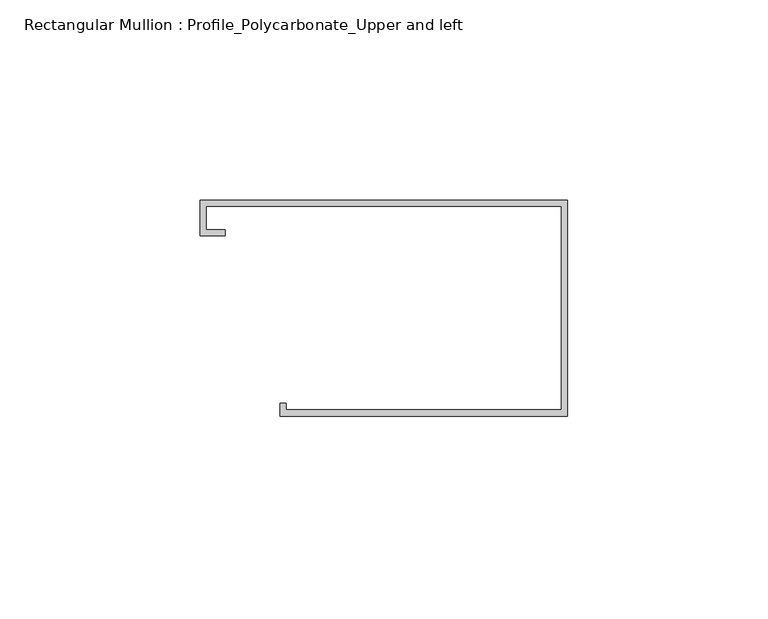
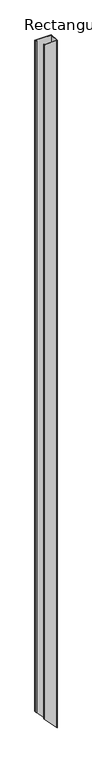
"""IFC4 building model written with IfcOpenShell, lengths in millimetres: member geometry, Rectangular Mullion : Profile_Polycarbonate_Upper and left."""

from ifc_helpers import new_model, si_unit, origin, place, context, project, spatial, faceted_brep, source, transform, mapped, element, save


def rectangular_mullion_profile_polycarbonate_upper_and_left_af227d46(model_context):
    return source(origin(), model_context, "Body", "Brep", [
        faceted_brep([(0.0, 28.984575, 0.0), (-91.9988, 28.984575, 0.0), (-91.9988, 19.992975, 0.0), (-85.6488, 19.992975, 0.0), (-85.6488, 21.580475, 0.0), (-90.4113, 21.580475, 0.0), (-90.4113, 27.397075, 0.0), (-1.5875, 27.397075, 0.0), (-1.5875, -23.428325, 0.0), (-70.3961, -23.428325, 0.0), (-70.3961, -21.840825, 0.0), (-71.9836, -21.840825, 0.0), (-71.9836, -25.015825, 0.0), (0.0, -25.015825, 0.0), (0.0, 28.984575, -4042.0750533), (-91.9988, 28.984575, -3946.1631445), (-91.9988, 19.992975, -3946.1631445), (-85.6488, 19.992975, -3952.7832376), (-85.6488, 21.580475, -3952.7832376), (-90.4113, 21.580475, -3947.8181678), (-90.4113, 27.397075, -3947.8181678), (-1.5875, 27.397075, -4040.42003), (-1.5875, -23.428325, -4040.42003), (-70.3961, -23.428325, -3968.6847012), (-70.3961, -21.840825, -3968.6847012), (-71.9836, -21.840825, -3967.029678), (-71.9836, -25.015825, -3967.029678), (0.0, -25.015825, -4042.0750533)], [[[0, 1, 2, 3, 4, 5, 6, 7, 8, 9, 10, 11, 12, 13]], [[1, 0, 14, 15]], [[2, 1, 15, 16]], [[3, 2, 16, 17]], [[4, 3, 17, 18]], [[5, 4, 18, 19]], [[6, 5, 19, 20]], [[7, 6, 20, 21]], [[8, 7, 21, 22]], [[9, 8, 22, 23]], [[10, 9, 23, 24]], [[11, 10, 24, 25]], [[12, 11, 25, 26]], [[13, 12, 26, 27]], [[0, 13, 27, 14]], [[14, 27, 26, 25, 24, 23, 22, 21, 20, 19, 18, 17, 16, 15]]]),
    ])


if __name__ == "__main__":
    model = new_model("IFC4")
    model_context = context("Model", 3, world=origin())
    ifc_project = project(units=[si_unit("LENGTHUNIT", "METRE", prefix="MILLI")], contexts=[model_context])
    site = spatial("IfcSite", under=ifc_project)
    building = spatial("IfcBuilding", under=site)
    placement = place(None, origin())
    rectangular_mullion_profile_polycarbonate_upper_and_left_shape = rectangular_mullion_profile_polycarbonate_upper_and_left_af227d46(model_context)
    element("IfcMember", 1, ObjectType="Rectangular Mullion : Profile_Polycarbonate_Upper and left", at=placement, inside=building, context=model_context, shape_type="MappedRepresentation", body=[
        mapped(rectangular_mullion_profile_polycarbonate_upper_and_left_shape, transform((0.0, 0.0, 0.0), x_axis=(1.0, 0.0, 0.0), y_axis=(0.0, 1.0, 0.0), z_axis=(0.0, 0.0, 1.0))),
    ])
    save(model, "model.ifc")

# Revit data of these elements
# Type "Rectangular Mullion : Profile_Polycarbonate_Upper and left"
#   built-in parameter 1007322 = 0.177167 (stored number, unit not read)
#   built-in parameter 1007321 = 0.00520833 (stored number, unit not read)
#   built-in parameter 1007320 = 0 (stored number, unit not read)
